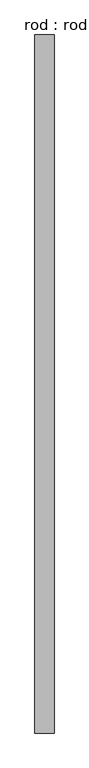
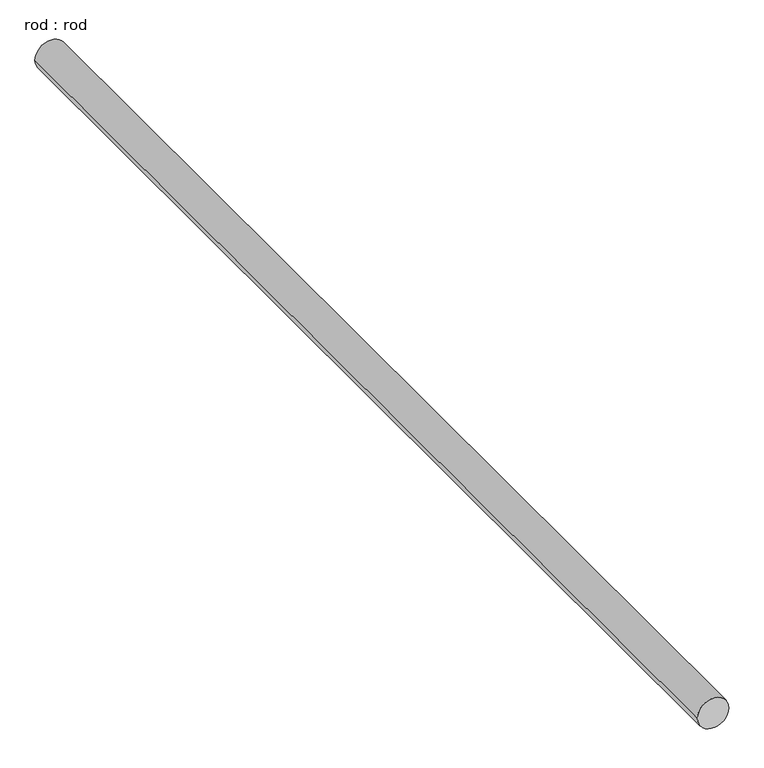
"""IFC4 building model written with IfcOpenShell, lengths in millimetres: proxy geometry, rod : rod."""

from ifc_helpers import new_model, si_unit, point, frame, frame_2d, origin, place, context, project, spatial, circle_curve, trimmed, segment, composite_curve, outline, extrude, source, transform, mapped, element, save


def rod_rod_a4141b39(model_context):
    return source(origin(), model_context, "Body", "SweptSolid", [
        extrude(outline(composite_curve([segment(trimmed(circle_curve(frame_2d((0.0108462, 0.0)), 200.0), [point((0.0108462, 200.0))], [point((0.0108462, -200.0))], False, "CARTESIAN"), True, "CONTINUOUS"), segment(trimmed(circle_curve(frame_2d((0.0108462, 0.0)), 200.0), [point((0.0108462, -200.0))], [point((0.0108462, 200.0))], False, "CARTESIAN"), True, "CONTINUOUS")], self_intersect=False)), frame((0.0, -3218.4964071, 0.0), z_axis=(0.0, 1.0, 0.0), x_axis=(0.0, 0.0, 1.0)), (0.0, 0.0, 1.0), 14622.4500448),
    ])


if __name__ == "__main__":
    model = new_model("IFC4")
    model_context = context("Model", 3, world=origin())
    ifc_project = project(units=[si_unit("LENGTHUNIT", "METRE", prefix="MILLI")], contexts=[model_context])
    site = spatial("IfcSite", under=ifc_project)
    building = spatial("IfcBuilding", under=site)
    placement = place(None, origin())
    rod_rod_shape = rod_rod_a4141b39(model_context)
    element("IfcBuildingElementProxy", 1, Name="rod : rod", ObjectType="rod : rod", at=placement, inside=building, context=model_context, shape_type="MappedRepresentation", body=[
        mapped(rod_rod_shape, transform((0.0, 0.0, 0.0), x_axis=(1.0, 0.0, 0.0), y_axis=(0.0, 1.0, 0.0), z_axis=(0.0, 0.0, 1.0))),
    ])
    save(model, "model.ifc")

# Revit data of these elements
# Type "rod : rod"
#   Default Elevation = 0
